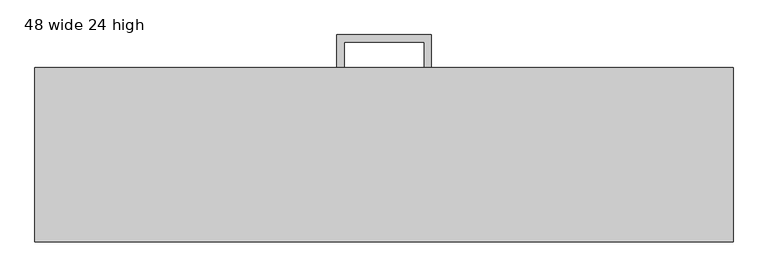
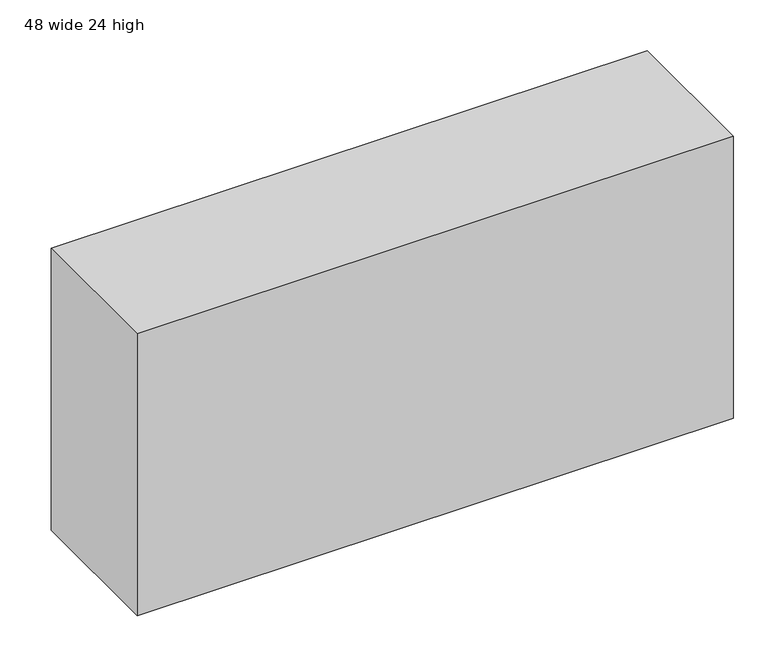
"""IFC4 building model written with IfcOpenShell, lengths in millimetres: furniture geometry, Binder Bin : 48 wide 24 high."""

import ifcopenshell
import ifcopenshell.guid

model = None  # the IFC model being written
_history = None  # IfcOwnerHistory: only IFC2X3 demands one
_inside = {}  # id of a spatial element -> (the spatial element, [elements in it])
_under = {}  # id of a project, library or spatial element -> (it, [spatial elements below it])
_declared = {}  # id of a project -> (the project, [libraries it declares])
_typed = {}  # id of a type object -> (the type object, [elements of that type])
_made_of = {}  # id of a material, layer set ... -> (it, [elements and type objects made of it])


def new_model(schema):
    """Start an empty IFC model of exactly this schema.

    Asked for "IFC4X3", IfcOpenShell would pick the latest addendum, in which some entities
    have other attributes; the version numbers below select the first issue.
    IFC2X3 requires an IfcOwnerHistory on every rooted entity: one is made here for all.
    """
    global model, _history
    if schema == "IFC4X3":
        model = ifcopenshell.file(schema_version=(4, 3, 0, 0))
    else:
        model = ifcopenshell.file(schema=schema)
    _inside.clear()
    _under.clear()
    _declared.clear()
    _typed.clear()
    _made_of.clear()
    _history = None
    if model.schema == "IFC2X3":
        org = make("IfcOrganization", Name="unknown")
        user = make(
            "IfcPersonAndOrganization",
            ThePerson=make("IfcPerson", FamilyName="unknown"),
            TheOrganization=org,
        )
        app = make(
            "IfcApplication",
            ApplicationDeveloper=org,
            Version="unknown",
            ApplicationFullName="unknown",
            ApplicationIdentifier="unknown",
        )
        _history = make(
            "IfcOwnerHistory",
            OwningUser=user,
            OwningApplication=app,
            ChangeAction="ADDED",
            CreationDate=0,
        )
    return model


def make(cls, **values):
    """One entity of the class cls with the attributes given. An attribute that is None is left unset."""
    return model.create_entity(
        cls, **{name: value for name, value in values.items() if value is not None}
    )


def rooted(cls, **values):
    """An entity with a GlobalId (a new one), such as an element, a storey or a relation."""
    return make(cls, GlobalId=ifcopenshell.guid.new(), OwnerHistory=_history, **values)


def si_unit(unit_type, name, prefix=None):
    """IfcSIUnit, for example si_unit("LENGTHUNIT", "METRE", prefix="MILLI")."""
    return make("IfcSIUnit", UnitType=unit_type, Prefix=prefix, Name=name)


def assignment(units):
    """IfcUnitAssignment: the units of a project."""
    return None if units is None else make("IfcUnitAssignment", Units=units)


def point(xyz):
    """IfcCartesianPoint."""
    return None if xyz is None else make("IfcCartesianPoint", Coordinates=xyz)


def direction(xyz):
    """IfcDirection."""
    return None if xyz is None else make("IfcDirection", DirectionRatios=xyz)


def frame(location, z_axis=None, x_axis=None):
    """IfcAxis2Placement3D, a coordinate frame: its origin and axes. An axis left out is left unset."""
    return make(
        "IfcAxis2Placement3D",
        Location=point(location),
        Axis=direction(z_axis),
        RefDirection=direction(x_axis),
    )


def origin():
    """The frame at (0, 0, 0) with its axes left unset."""
    return frame((0.0, 0.0, 0.0))


def place(relative_to, where):
    """IfcLocalPlacement: puts the frame where relative to a parent placement (None: the world)."""
    return make(
        "IfcLocalPlacement", PlacementRelTo=relative_to, RelativePlacement=where
    )


def context(
    kind, dimensions, precision=None, world=None, true_north=None, identifier=None
):
    """IfcGeometricRepresentationContext, for example the 3D "Model" context."""
    return make(
        "IfcGeometricRepresentationContext",
        ContextIdentifier=identifier,
        ContextType=kind,
        CoordinateSpaceDimension=dimensions,
        Precision=precision,
        WorldCoordinateSystem=world,
        TrueNorth=true_north,
    )


def project(units=None, contexts=None):
    """IfcProject with its units and contexts."""
    return rooted(
        "IfcProject",
        Name="project",
        RepresentationContexts=contexts,
        UnitsInContext=assignment(units),
    )


def spatial(cls, under=None, at=None, **own):
    """A site, building, storey or space (cls), placed at a placement, below another one or the project."""
    s = rooted(cls, ObjectPlacement=at, **own)
    if under is not None:
        _under.setdefault(under.id(), (under, []))[1].append(s)
    return s


def polyline(points):
    """IfcPolyline through the points."""
    return make("IfcPolyline", Points=[point(p) for p in points])


def outline(outer, holes=None, kind="AREA"):
    """IfcArbitraryClosedProfileDef: a profile drawn as a closed curve; with holes, ...WithVoids."""
    if holes is None:
        return make("IfcArbitraryClosedProfileDef", ProfileType=kind, OuterCurve=outer)
    return make(
        "IfcArbitraryProfileDefWithVoids",
        ProfileType=kind,
        OuterCurve=outer,
        InnerCurves=holes,
    )


def extrude(swept, where, along, depth):
    """IfcExtrudedAreaSolid: the profile swept, set in the frame where, extruded along a direction by depth."""
    return make(
        "IfcExtrudedAreaSolid",
        SweptArea=swept,
        Position=where,
        ExtrudedDirection=direction(along),
        Depth=depth,
    )


def shape(context_of_items, identifier, shape_type, items):
    """IfcShapeRepresentation: the items that make up one representation, for example the "Body"."""
    return make(
        "IfcShapeRepresentation",
        ContextOfItems=context_of_items,
        RepresentationIdentifier=identifier,
        RepresentationType=shape_type,
        Items=items,
    )


def source(mapping_origin, context_of_items, identifier, shape_type, items):
    """IfcRepresentationMap: a shape defined once, which mapped items show again and again."""
    return make(
        "IfcRepresentationMap",
        MappingOrigin=mapping_origin,
        MappedRepresentation=shape(context_of_items, identifier, shape_type, items),
    )


def transform(
    local_origin,
    x_axis=None,
    y_axis=None,
    z_axis=None,
    scale=None,
    scale2=None,
    scale3=None,
    uniform=True,
):
    """IfcCartesianTransformationOperator3D, or its non-uniform kind. x_axis, y_axis, z_axis: its Axis1, 2, 3."""
    if uniform:
        return make(
            "IfcCartesianTransformationOperator3D",
            Axis1=direction(x_axis),
            Axis2=direction(y_axis),
            LocalOrigin=point(local_origin),
            Scale=scale,
            Axis3=direction(z_axis),
        )
    return make(
        "IfcCartesianTransformationOperator3DnonUniform",
        Axis1=direction(x_axis),
        Axis2=direction(y_axis),
        LocalOrigin=point(local_origin),
        Scale=scale,
        Axis3=direction(z_axis),
        Scale2=scale2,
        Scale3=scale3,
    )


def mapped(mapping_source, mapping_target):
    """IfcMappedItem: shows the shape of a source again, moved by a transform."""
    return make(
        "IfcMappedItem", MappingSource=mapping_source, MappingTarget=mapping_target
    )


def made_of(thing, what):
    """Note that an element or type object is made of a material, layer set ...; save() writes the relation."""
    if what is not None:
        _made_of.setdefault(what.id(), (what, []))[1].append(thing)
    return thing


def element(
    cls,
    number,
    at=None,
    inside=None,
    cuts=None,
    type_object=None,
    material=None,
    context=None,
    identifier="Body",
    shape_type=None,
    held_by="IfcProductDefinitionShape",
    body=None,
    shapes=None,
    **own,
):
    """One element of the class cls, such as IfcWall. Its Tag is "e" and its number.

    at: its placement. inside: the storey or other place that contains it. cuts: it is an
    opening in that element (IfcRelVoidsElement). A single representation is given by context,
    identifier, shape_type and body (its items); several are given by shapes. held_by: the class
    of the entity that holds the representations. save() writes the other relations.
    """
    e = rooted(cls, Tag="e%d" % number, ObjectPlacement=at, **own)
    if body is not None:
        shapes = [shape(context, identifier, shape_type, body)]
    if shapes is not None:
        e.Representation = make(held_by, Representations=shapes)
    if inside is not None:
        _inside.setdefault(inside.id(), (inside, []))[1].append(e)
    if cuts is not None:
        rooted(
            "IfcRelVoidsElement", RelatingBuildingElement=cuts, RelatedOpeningElement=e
        )
    if type_object is not None:
        _typed.setdefault(type_object.id(), (type_object, []))[1].append(e)
    return made_of(e, material)


def aggregate(whole, parts):
    """IfcRelAggregates: a whole, such as a stair, and the parts it consists of."""
    return rooted("IfcRelAggregates", RelatingObject=whole, RelatedObjects=parts)


def save(model, path):
    """Write the relations noted so far, then the file.

    IfcRelAggregates (storeys below a building ...), IfcRelContainedInSpatialStructure (elements
    in a storey), IfcRelDefinesByType, IfcRelAssociatesMaterial and IfcRelDeclares: one each for
    every whole, place, type object, material and project.
    """
    for whole, parts in _under.values():
        aggregate(whole, parts)
    for where, things in _inside.values():
        rooted(
            "IfcRelContainedInSpatialStructure",
            RelatedElements=things,
            RelatingStructure=where,
        )
    for kind, things in _typed.values():
        rooted("IfcRelDefinesByType", RelatedObjects=things, RelatingType=kind)
    for what, things in _made_of.values():
        rooted("IfcRelAssociatesMaterial", RelatedObjects=things, RelatingMaterial=what)
    for by, libraries in _declared.values():
        rooted("IfcRelDeclares", RelatingContext=by, RelatedDefinitions=libraries)
    model.write(path)


def furniture_48_wide_24_high_fb19277b(model_context):
    return source(origin(), model_context, "Body", "SweptSolid", [
        extrude(outline(polyline([(-69.85, 381.0), (-82.55, 381.0), (-82.55, 438.15), (82.55, 438.15), (82.55, 381.0), (69.85, 381.0), (69.85, 425.45), (-69.85, 425.45), (-69.85, 381.0)])), frame((0.0, 0.0, 1416.05), z_axis=(0.0, 0.0, 1.0), x_axis=(1.0, 0.0, 0.0)), (0.0, 0.0, 1.0), 12.7),
        extrude(outline(polyline([(609.6, 76.2), (-609.6, 76.2), (-609.6, 381.0), (609.6, 381.0), (609.6, 76.2)])), frame((0.0, 0.0, 1371.6), z_axis=(0.0, 0.0, 1.0), x_axis=(1.0, 0.0, 0.0)), (0.0, 0.0, 1.0), 609.6),
    ])


if __name__ == "__main__":
    model = new_model("IFC4")
    model_context = context("Model", 3, world=origin())
    ifc_project = project(units=[si_unit("LENGTHUNIT", "METRE", prefix="MILLI")], contexts=[model_context])
    site = spatial("IfcSite", under=ifc_project)
    building = spatial("IfcBuilding", under=site)
    placement = place(None, origin())
    furniture_48_wide_24_high_shape = furniture_48_wide_24_high_fb19277b(model_context)
    element("IfcFurniture", 1, ObjectType="Binder Bin : 48 wide 24 high", at=placement, inside=building, context=model_context, shape_type="MappedRepresentation", body=[
        mapped(furniture_48_wide_24_high_shape, transform((0.0, 0.0, 0.0), x_axis=(1.0, 0.0, 0.0), y_axis=(0.0, 1.0, 0.0), z_axis=(0.0, 0.0, 1.0))),
    ])
    save(model, "model.ifc")

# Revit data of these elements
# Type "Binder Bin : 48 wide 24 high"
#   Model = "BIN-4824"
#   Manufacturer = "Corporate Concepts"
#   Type Mark = "BN-3"
#   Model = "BIN-4824"
#   Manufacturer = "Corporate Concepts"
#   Cost = 785
#   Width = 4' - 0"
#   Mounting Height [instance default] = 4' - 6"
#   Height = 2' - 0"
#   Cost = 785
#   Type Image = Binder Bin.png
#   Default Elevation = 0
